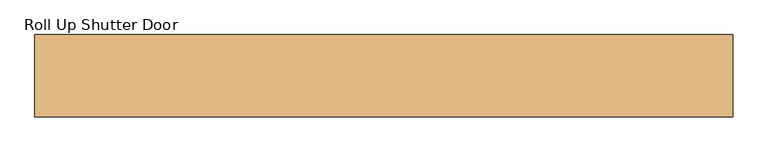
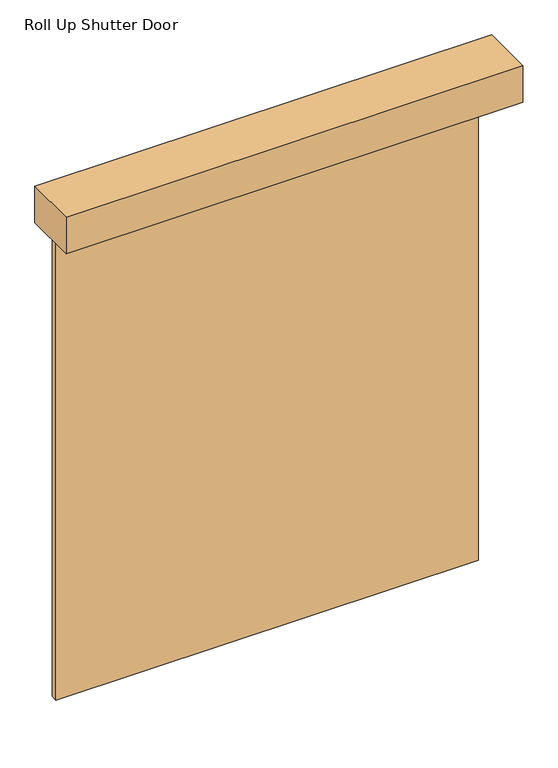
"""IFC4 building model written with IfcOpenShell, lengths in millimetres: door geometry, Roll Up Shutter Door : H_DR_AMD_Steel Rollup Shutter_W5000xH6000."""

from ifc_helpers import new_model, si_unit, frame, origin, origin_with_axes, place, context, project, spatial, polyline, outline, extrude, source, transform, mapped, element, save


def roll_up_shutter_door_e99b7ff9(model_context):
    return source(origin(), model_context, "Body", "SweptSolid", [
        extrude(outline(polyline([(2703.2, -858.8), (-2703.2, -858.8), (-2703.2, -220.0), (2703.2, -220.0), (2703.2, -858.8)])), frame((0.0, 0.0, 6000.0), z_axis=(0.0, 0.0, 1.0), x_axis=(1.0, 0.0, 0.0)), (0.0, 0.0, 1.0), 457.2),
        extrude(outline(polyline([(2500.0, -220.0), (2500.0, -300.0), (-2500.0, -300.0), (-2500.0, -220.0), (2500.0, -220.0)])), origin_with_axes(), (0.0, 0.0, 1.0), 6000.0),
    ])


if __name__ == "__main__":
    model = new_model("IFC4")
    model_context = context("Model", 3, world=origin())
    ifc_project = project(units=[si_unit("LENGTHUNIT", "METRE", prefix="MILLI")], contexts=[model_context])
    site = spatial("IfcSite", under=ifc_project)
    building = spatial("IfcBuilding", under=site)
    placement = place(None, origin())
    roll_up_shutter_door_shape = roll_up_shutter_door_e99b7ff9(model_context)
    element("IfcDoor", 1, ObjectType="Roll Up Shutter Door : H_DR_AMD_Steel Rollup Shutter_W5000xH6000", at=placement, inside=building, context=model_context, shape_type="MappedRepresentation", body=[
        mapped(roll_up_shutter_door_shape, transform((0.0, 0.0, 0.0), x_axis=(1.0, 0.0, 0.0), y_axis=(0.0, 1.0, 0.0), z_axis=(0.0, 0.0, 1.0))),
    ])
    save(model, "model.ifc")

# Revit data of these elements
# Type "Roll Up Shutter Door : H_DR_AMD_Steel Rollup Shutter_W5000xH6000"
#   Type Mark = "RD"
#   H_WM Code_1 = "A04AR127-00001 | Finishing Work | Door & Window Work | Steel Roll Up Door w/ Steel Frame (UoM: EA) | Fire Protective Rating: N/A, Motorized Type | w/ Hardware & Accessories | W x H=(  )mm x (  )mm"
#   H_Q'ty Cal Type Tag = "DR-Q1"
#   Construction Type Id = "MDOOR"
#   Assembly Code = "B2030400"
#   Analytic Construction = "<None>"
#   Thickness = 0.0800 m
#   Thermal Resistance (R) = 0.270117 (m²·K)/W
#   Rough Width [instance default] = 4.0000 m
#   Rough Height [instance default] = 4.0000 m
#   Offset [instance default] = 1.0000 m
#   Heat Transfer Coefficient (U) = 3.7021 W/(m²·K)
#   Height [instance default] = 4.0000 m
#   Width [instance default] = 4.0000 m
#   Function = 1
#   Define Thermal Properties by = 1
#   Canopy [instance default] = yes
#   Roller Material = A04AQ112-00002_Steel Roll Up Door
#   Roller Box Material = A04AQ112-00002_Steel Roll Up Door
#   Visual Light Transmittance = 0
#   Solar Heat Gain Coefficient = 0
#   Wall Closure = (empty or 0)
# Element 1 (IfcDoor, "Roll Up Shutter Door : H_DR_AMD_Steel Rollup Shutter_W5000xH6000")
#   Rough Width = 5.0000 m
#   Rough Height = 6.0000 m
#   Offset = 0.2600 m
#   Height = 6.0000 m
#   Width = 5.0000 m
#   Canopy = no
#   Materials on its faces: "A04AQ112-00002_Steel Roll Up Door"
# Materials
#   "A04AQ112-00002_Steel Roll Up Door": class "금속", colour RGB 247 247 247, transparency 0, Description = "Steel Door", Cost = 0
